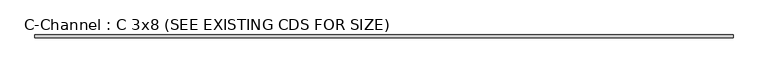
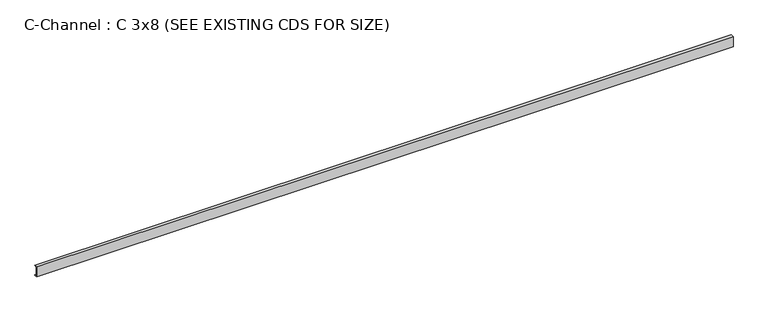
"""IFC4 building model written with IfcOpenShell, lengths in millimetres: beam geometry, C-Channel : C 3x8 (SEE EXISTING CDS FOR SIZE)."""

from ifc_helpers import new_model, si_unit, point, frame, frame_2d, origin, place, context, project, spatial, polyline, circle_curve, trimmed, segment, composite_curve, outline, extrude, source, transform, mapped, element, save


def c_channel_c_3x8_see_existing_cds_for_size_a37141a3(model_context):
    return source(origin(), model_context, "Body", "SweptSolid", [
        extrude(outline(composite_curve([segment(polyline([(-13.5128, 101.6), (44.9072, 101.6)]), True, "CONTINUOUS"), segment(trimmed(circle_curve(frame_2d((35.6108, 101.6)), 9.2964), [point((44.9072, 101.6))], [point((35.6108, 92.3036))], False, "CARTESIAN"), True, "CONTINUOUS"), segment(polyline([(35.6108, 92.3036), (-2.8702, 86.2088084), (-2.8702, -86.2088084), (35.6108, -92.3036)]), True, "CONTINUOUS"), segment(trimmed(circle_curve(frame_2d((35.6108, -101.6)), 9.2964), [point((35.6108, -92.3036))], [point((44.9072, -101.6))], False, "CARTESIAN"), True, "CONTINUOUS"), segment(polyline([(44.9072, -101.6), (-13.5128, -101.6), (-13.5128, 101.6)]), True, "CONTINUOUS")], self_intersect=False)), frame((-6696.075, 0.0, 0.0), z_axis=(1.0, 0.0, 0.0), x_axis=(0.0, 1.0, 0.0)), (0.0, 0.0, 1.0), 13392.1499994),
    ])


if __name__ == "__main__":
    model = new_model("IFC4")
    model_context = context("Model", 3, world=origin())
    ifc_project = project(units=[si_unit("LENGTHUNIT", "METRE", prefix="MILLI")], contexts=[model_context])
    site = spatial("IfcSite", under=ifc_project)
    building = spatial("IfcBuilding", under=site)
    placement = place(None, origin())
    c_channel_c_3x8_see_existing_cds_for_size_shape = c_channel_c_3x8_see_existing_cds_for_size_a37141a3(model_context)
    element("IfcBeam", 1, ObjectType="C-Channel : C 3x8 (SEE EXISTING CDS FOR SIZE)", at=placement, inside=building, context=model_context, shape_type="MappedRepresentation", body=[
        mapped(c_channel_c_3x8_see_existing_cds_for_size_shape, transform((0.0, 0.0, 0.0), x_axis=(1.0, 0.0, 0.0), y_axis=(0.0, 1.0, 0.0), z_axis=(0.0, 0.0, 1.0))),
    ])
    save(model, "model.ifc")

# Revit data of these elements
# Type "C-Channel : C 3x8 (SEE EXISTING CDS FOR SIZE)"
#   Assembly Code = "B10"
#   W = 14.7
#   Length [instance default] = 5' - 0"
#   bf = 0' - 2.3"
#   d = 0' - 8"
#   tf = 0' - 0.366"
#   tw = 0' - 0.419"
#   x = 0' - 0.532"
#   A = 0.0300694 SF
#   Structural Material [instance default] = Steel ASTM A36
# Element 1 (IfcBeam, "C-Channel : C 3x8 (SEE EXISTING CDS FOR SIZE)")
#   Structural Material = Steel ASTM A992
#   Materials on its faces: "Steel ASTM A992"
# Materials
#   "Steel ASTM A36": class "Metal", colour RGB 199 199 199, transparency 0, Description = "Structural steel, ASTM A36 Grade B, mill finish", Cost = 0
#   "Steel ASTM A992": class "Metal", colour RGB 189 187 185, transparency 0, Description = "Structural steel 50ksi", Cost = 0
